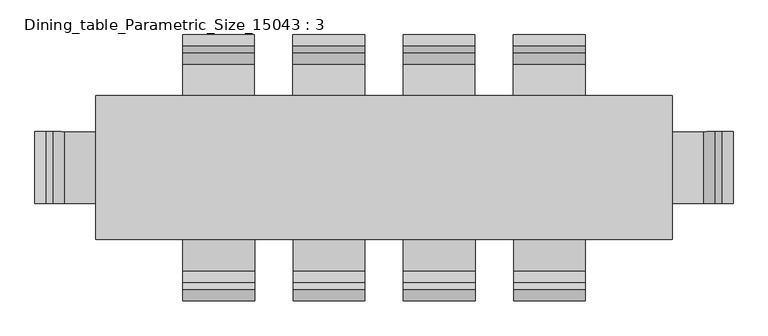
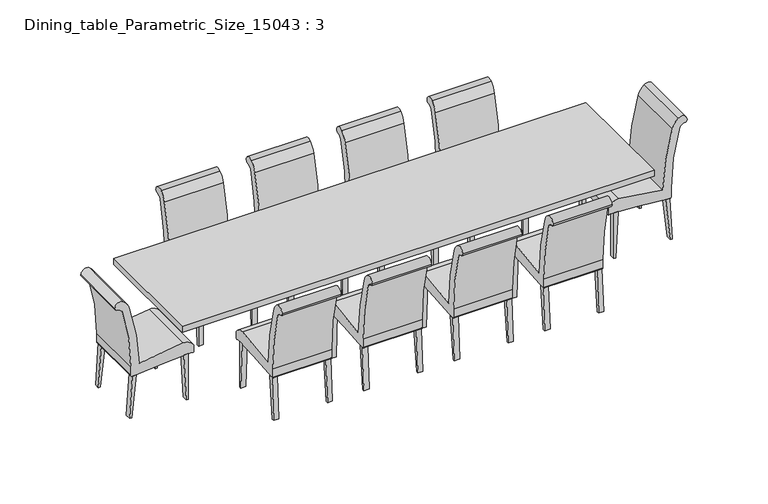
"""IFC4 building model written with IfcOpenShell, lengths in millimetres: furniture geometry, Dining_table_Parametric_Size_15043 : 3."""

from ifc_helpers import new_model, si_unit, point, frame, frame_2d, origin, place, context, project, spatial, polyline, circle_curve, trimmed, segment, composite_curve, outline, extrude, source, transform, mapped, element, save


def dining_table_parametric_size_15043_3_5ca9b808(model_context):
    return source(origin(), model_context, "Body", "SweptSolid", [
        extrude(outline(polyline([(-292.8098174, 0.0), (-312.156828, 373.7391541), (-276.8521088, 373.7391541), (-276.8521088, 0.0), (-292.8098174, 0.0)])), frame((821.4, 0.0, 0.0), z_axis=(1.0, 0.0, 0.0), x_axis=(0.0, 1.0, 0.0)), (0.0, 0.0, 1.0), 38.1),
        extrude(outline(composite_curve([segment(polyline([(-710.0841698, 339.961294), (-678.3341698, 339.961294)]), True, "CONTINUOUS"), segment(trimmed(circle_curve(frame_2d((-4714.5831391, 601.3302132)), 4044.702641), [point((-678.3341698, 339.961294))], [point((-714.8304681, 0.0))], False, "CARTESIAN"), True, "CONTINUOUS"), segment(polyline([(-714.8304681, 0.0), (-730.8247987, 0.0)]), True, "CONTINUOUS"), segment(trimmed(circle_curve(frame_2d((-4796.627411, 418.6630455)), 4087.30102), [point((-730.8247987, 0.0))], [point((-710.0841698, 339.961294))], True, "CARTESIAN"), True, "CONTINUOUS")], self_intersect=False)), frame((822.7642545, 0.0, 0.0), z_axis=(1.0, 0.0, 0.0), x_axis=(0.0, 1.0, 0.0)), (0.0, 0.0, 1.0), 41.6791394),
        extrude(outline(polyline([(-290.2637156, 0.0), (-309.6107262, 373.7391541), (-274.306007, 373.7391541), (-274.306007, 0.0), (-290.2637156, 0.0)])), frame((1240.5, 0.0, 0.0), z_axis=(1.0, 0.0, 0.0), x_axis=(0.0, 1.0, 0.0)), (0.0, 0.0, 1.0), 38.1),
        extrude(outline(composite_curve([segment(polyline([(-710.2334533, 339.961294), (-678.4834533, 339.961294)]), True, "CONTINUOUS"), segment(trimmed(circle_curve(frame_2d((-4714.7324226, 601.3302132)), 4044.702641), [point((-678.4834533, 339.961294))], [point((-714.9797517, 0.0))], False, "CARTESIAN"), True, "CONTINUOUS"), segment(polyline([(-714.9797517, 0.0), (-730.9740822, 0.0)]), True, "CONTINUOUS"), segment(trimmed(circle_curve(frame_2d((-4796.7766946, 418.6630455)), 4087.30102), [point((-730.9740822, 0.0))], [point((-710.2334533, 339.961294))], True, "CARTESIAN"), True, "CONTINUOUS")], self_intersect=False)), frame((1240.5, 0.0, 0.0), z_axis=(1.0, 0.0, 0.0), x_axis=(0.0, 1.0, 0.0)), (0.0, 0.0, 1.0), 38.1),
        extrude(outline(composite_curve([segment(trimmed(circle_curve(frame_2d((-2455.1641625, 418.9322486)), 1733.8120537), [point((-721.3521088, 418.9322486))], [point((-788.5170473, 896.8356186))], True, "CARTESIAN"), True, "CONTINUOUS"), segment(trimmed(circle_curve(frame_2d((-836.5595379, 866.2613731)), 56.9461622), [point((-788.5170473, 896.8356186))], [point((-833.5560291, 923.1282732))], True, "CARTESIAN"), True, "CONTINUOUS"), segment(trimmed(circle_curve(frame_2d((-822.9723933, 942.5682988)), 22.134316), [point((-833.5560291, 923.1282732))], [point((-845.0415591, 944.2653155))], False, "CARTESIAN"), True, "CONTINUOUS"), segment(trimmed(circle_curve(frame_2d((-802.9630897, 941.029676)), 42.2026889), [point((-845.0415591, 944.2653155))], [point((-776.060453, 973.5460579))], False, "CARTESIAN"), True, "CONTINUOUS"), segment(trimmed(circle_curve(frame_2d((-859.9657861, 872.1322861)), 131.6239265), [point((-776.060453, 973.5460579))], [point((-732.0340147, 903.0890285))], False, "CARTESIAN"), True, "CONTINUOUS"), segment(trimmed(circle_curve(frame_2d((-2494.3548845, 379.656989)), 1838.4112565), [point((-732.0340147, 903.0890285))], [point((-656.5387419, 426.4306353))], False, "CARTESIAN"), True, "CONTINUOUS"), segment(trimmed(circle_curve(frame_2d((-123.3478444, -2135.5006423)), 2616.8271636), [point((-656.5387419, 426.4306353))], [point((-316.9758211, 474.1530916))], False, "CARTESIAN"), True, "CONTINUOUS"), segment(trimmed(circle_curve(frame_2d((-310.4852539, 386.6753768)), 87.718174), [point((-316.9758211, 474.1530916))], [point((-232.8604678, 427.5271899))], False, "CARTESIAN"), True, "CONTINUOUS"), segment(polyline([(-232.8604678, 427.5271899), (-232.8604678, 371.8464813), (-237.3505959, 367.3563533), (-247.15219, 373.0153063)]), True, "CONTINUOUS"), segment(trimmed(circle_curve(frame_2d((-291.8347617, -793.4944233)), 1167.3651877), [point((-247.15219, 373.0153063))], [point((-457.2, 362.0988526))], True, "CARTESIAN"), True, "CONTINUOUS"), segment(trimmed(circle_curve(frame_2d((-785.2472905, 2654.5349591)), 2315.7889211), [point((-457.2, 362.0988526))], [point((-710.2334533, 339.961294))], False, "CARTESIAN"), True, "CONTINUOUS"), segment(trimmed(circle_curve(frame_2d((-712.0516896, 349.0822486)), 9.3004191), [point((-710.2334533, 339.961294))], [point((-721.3521088, 349.0822486))], False, "CARTESIAN"), True, "CONTINUOUS"), segment(polyline([(-721.3521088, 349.0822486), (-721.3521088, 418.9322486)]), True, "CONTINUOUS")], self_intersect=False)), frame((822.7642545, 0.0, 0.0), z_axis=(1.0, 0.0, 0.0), x_axis=(0.0, 1.0, 0.0)), (0.0, 0.0, 1.0), 455.8357455),
        extrude(outline(polyline([(-292.8098174, 0.0), (-312.156828, 373.7391541), (-276.8521088, 373.7391541), (-276.8521088, 0.0), (-292.8098174, 0.0)])), frame((121.4, 0.0, 0.0), z_axis=(1.0, 0.0, 0.0), x_axis=(0.0, 1.0, 0.0)), (0.0, 0.0, 1.0), 38.1),
        extrude(outline(composite_curve([segment(polyline([(-710.0841698, 339.961294), (-678.3341698, 339.961294)]), True, "CONTINUOUS"), segment(trimmed(circle_curve(frame_2d((-4714.5831391, 601.3302132)), 4044.702641), [point((-678.3341698, 339.961294))], [point((-714.8304681, 0.0))], False, "CARTESIAN"), True, "CONTINUOUS"), segment(polyline([(-714.8304681, 0.0), (-730.8247987, 0.0)]), True, "CONTINUOUS"), segment(trimmed(circle_curve(frame_2d((-4796.627411, 418.6630455)), 4087.30102), [point((-730.8247987, 0.0))], [point((-710.0841698, 339.961294))], True, "CARTESIAN"), True, "CONTINUOUS")], self_intersect=False)), frame((122.7642545, 0.0, 0.0), z_axis=(1.0, 0.0, 0.0), x_axis=(0.0, 1.0, 0.0)), (0.0, 0.0, 1.0), 41.6791394),
        extrude(outline(polyline([(-290.2637156, 0.0), (-309.6107262, 373.7391541), (-274.306007, 373.7391541), (-274.306007, 0.0), (-290.2637156, 0.0)])), frame((540.5, 0.0, 0.0), z_axis=(1.0, 0.0, 0.0), x_axis=(0.0, 1.0, 0.0)), (0.0, 0.0, 1.0), 38.1),
        extrude(outline(composite_curve([segment(polyline([(-710.2334533, 339.961294), (-678.4834533, 339.961294)]), True, "CONTINUOUS"), segment(trimmed(circle_curve(frame_2d((-4714.7324226, 601.3302132)), 4044.702641), [point((-678.4834533, 339.961294))], [point((-714.9797517, 0.0))], False, "CARTESIAN"), True, "CONTINUOUS"), segment(polyline([(-714.9797517, 0.0), (-730.9740822, 0.0)]), True, "CONTINUOUS"), segment(trimmed(circle_curve(frame_2d((-4796.7766946, 418.6630455)), 4087.30102), [point((-730.9740822, 0.0))], [point((-710.2334533, 339.961294))], True, "CARTESIAN"), True, "CONTINUOUS")], self_intersect=False)), frame((540.5, 0.0, 0.0), z_axis=(1.0, 0.0, 0.0), x_axis=(0.0, 1.0, 0.0)), (0.0, 0.0, 1.0), 38.1),
        extrude(outline(composite_curve([segment(trimmed(circle_curve(frame_2d((-2455.1641625, 418.9322486)), 1733.8120537), [point((-721.3521088, 418.9322486))], [point((-788.5170473, 896.8356186))], True, "CARTESIAN"), True, "CONTINUOUS"), segment(trimmed(circle_curve(frame_2d((-836.5595379, 866.2613731)), 56.9461622), [point((-788.5170473, 896.8356186))], [point((-833.5560291, 923.1282732))], True, "CARTESIAN"), True, "CONTINUOUS"), segment(trimmed(circle_curve(frame_2d((-822.9723933, 942.5682988)), 22.134316), [point((-833.5560291, 923.1282732))], [point((-845.0415591, 944.2653155))], False, "CARTESIAN"), True, "CONTINUOUS"), segment(trimmed(circle_curve(frame_2d((-802.9630897, 941.029676)), 42.2026889), [point((-845.0415591, 944.2653155))], [point((-776.060453, 973.5460579))], False, "CARTESIAN"), True, "CONTINUOUS"), segment(trimmed(circle_curve(frame_2d((-859.9657861, 872.1322861)), 131.6239265), [point((-776.060453, 973.5460579))], [point((-732.0340147, 903.0890285))], False, "CARTESIAN"), True, "CONTINUOUS"), segment(trimmed(circle_curve(frame_2d((-2494.3548845, 379.656989)), 1838.4112565), [point((-732.0340147, 903.0890285))], [point((-656.5387419, 426.4306353))], False, "CARTESIAN"), True, "CONTINUOUS"), segment(trimmed(circle_curve(frame_2d((-123.3478444, -2135.5006423)), 2616.8271636), [point((-656.5387419, 426.4306353))], [point((-316.9758211, 474.1530916))], False, "CARTESIAN"), True, "CONTINUOUS"), segment(trimmed(circle_curve(frame_2d((-310.4852539, 386.6753768)), 87.718174), [point((-316.9758211, 474.1530916))], [point((-232.8604678, 427.5271899))], False, "CARTESIAN"), True, "CONTINUOUS"), segment(polyline([(-232.8604678, 427.5271899), (-232.8604678, 371.8464813), (-237.3505959, 367.3563533), (-247.15219, 373.0153063)]), True, "CONTINUOUS"), segment(trimmed(circle_curve(frame_2d((-291.8347617, -793.4944233)), 1167.3651877), [point((-247.15219, 373.0153063))], [point((-457.2, 362.0988526))], True, "CARTESIAN"), True, "CONTINUOUS"), segment(trimmed(circle_curve(frame_2d((-785.2472905, 2654.5349591)), 2315.7889211), [point((-457.2, 362.0988526))], [point((-710.2334533, 339.961294))], False, "CARTESIAN"), True, "CONTINUOUS"), segment(trimmed(circle_curve(frame_2d((-712.0516896, 349.0822486)), 9.3004191), [point((-710.2334533, 339.961294))], [point((-721.3521088, 349.0822486))], False, "CARTESIAN"), True, "CONTINUOUS"), segment(polyline([(-721.3521088, 349.0822486), (-721.3521088, 418.9322486)]), True, "CONTINUOUS")], self_intersect=False)), frame((122.7642545, 0.0, 0.0), z_axis=(1.0, 0.0, 0.0), x_axis=(0.0, 1.0, 0.0)), (0.0, 0.0, 1.0), 455.8357455),
        extrude(outline(polyline([(292.8098174, 0.0), (276.8521088, 0.0), (276.8521088, 373.7391541), (312.156828, 373.7391541), (292.8098174, 0.0)])), frame((1240.5, 0.0, 0.0), z_axis=(1.0, 0.0, 0.0), x_axis=(0.0, 1.0, 0.0)), (0.0, 0.0, 1.0), 38.1),
        extrude(outline(composite_curve([segment(trimmed(circle_curve(frame_2d((4796.627411, 418.6630455)), 4087.30102), [point((710.0841698, 339.961294))], [point((730.8247987, 0.0))], True, "CARTESIAN"), True, "CONTINUOUS"), segment(polyline([(730.8247987, 0.0), (714.8304681, 0.0)]), True, "CONTINUOUS"), segment(trimmed(circle_curve(frame_2d((4714.5831391, 601.3302132)), 4044.702641), [point((714.8304681, 0.0))], [point((678.3341698, 339.961294))], False, "CARTESIAN"), True, "CONTINUOUS"), segment(polyline([(678.3341698, 339.961294), (710.0841698, 339.961294)]), True, "CONTINUOUS")], self_intersect=False)), frame((1235.5566061, 0.0, 0.0), z_axis=(1.0, 0.0, 0.0), x_axis=(0.0, 1.0, 0.0)), (0.0, 0.0, 1.0), 41.6791394),
        extrude(outline(polyline([(290.2637156, 0.0), (274.306007, 0.0), (274.306007, 373.7391541), (309.6107262, 373.7391541), (290.2637156, 0.0)])), frame((821.4, 0.0, 0.0), z_axis=(1.0, 0.0, 0.0), x_axis=(0.0, 1.0, 0.0)), (0.0, 0.0, 1.0), 38.1),
        extrude(outline(composite_curve([segment(trimmed(circle_curve(frame_2d((4796.7766946, 418.6630455)), 4087.30102), [point((710.2334533, 339.961294))], [point((730.9740822, 0.0))], True, "CARTESIAN"), True, "CONTINUOUS"), segment(polyline([(730.9740822, 0.0), (714.9797517, 0.0)]), True, "CONTINUOUS"), segment(trimmed(circle_curve(frame_2d((4714.7324226, 601.3302132)), 4044.702641), [point((714.9797517, 0.0))], [point((678.4834533, 339.961294))], False, "CARTESIAN"), True, "CONTINUOUS"), segment(polyline([(678.4834533, 339.961294), (710.2334533, 339.961294)]), True, "CONTINUOUS")], self_intersect=False)), frame((821.4, 0.0, 0.0), z_axis=(1.0, 0.0, 0.0), x_axis=(0.0, 1.0, 0.0)), (0.0, 0.0, 1.0), 38.1),
        extrude(outline(composite_curve([segment(polyline([(721.3521088, 418.9322486), (721.3521088, 349.0822486)]), True, "CONTINUOUS"), segment(trimmed(circle_curve(frame_2d((712.0516896, 349.0822486)), 9.3004191), [point((721.3521088, 349.0822486))], [point((710.2334533, 339.961294))], False, "CARTESIAN"), True, "CONTINUOUS"), segment(trimmed(circle_curve(frame_2d((785.2472905, 2654.5349591)), 2315.7889211), [point((710.2334533, 339.961294))], [point((457.2, 362.0988526))], False, "CARTESIAN"), True, "CONTINUOUS"), segment(trimmed(circle_curve(frame_2d((291.8347617, -793.4944233)), 1167.3651877), [point((457.2, 362.0988526))], [point((247.15219, 373.0153063))], True, "CARTESIAN"), True, "CONTINUOUS"), segment(polyline([(247.15219, 373.0153063), (237.3505959, 367.3563533), (232.8604678, 371.8464813), (232.8604678, 427.5271899)]), True, "CONTINUOUS"), segment(trimmed(circle_curve(frame_2d((310.4852539, 386.6753768)), 87.718174), [point((232.8604678, 427.5271899))], [point((316.9758211, 474.1530916))], False, "CARTESIAN"), True, "CONTINUOUS"), segment(trimmed(circle_curve(frame_2d((123.3478444, -2135.5006423)), 2616.8271636), [point((316.9758211, 474.1530916))], [point((656.5387419, 426.4306353))], False, "CARTESIAN"), True, "CONTINUOUS"), segment(trimmed(circle_curve(frame_2d((2494.3548845, 379.656989)), 1838.4112565), [point((656.5387419, 426.4306353))], [point((732.0340147, 903.0890285))], False, "CARTESIAN"), True, "CONTINUOUS"), segment(trimmed(circle_curve(frame_2d((859.9657861, 872.1322861)), 131.6239265), [point((732.0340147, 903.0890285))], [point((776.060453, 973.5460579))], False, "CARTESIAN"), True, "CONTINUOUS"), segment(trimmed(circle_curve(frame_2d((802.9630897, 941.029676)), 42.2026889), [point((776.060453, 973.5460579))], [point((845.0415591, 944.2653155))], False, "CARTESIAN"), True, "CONTINUOUS"), segment(trimmed(circle_curve(frame_2d((822.9723933, 942.5682988)), 22.134316), [point((845.0415591, 944.2653155))], [point((833.5560291, 923.1282732))], False, "CARTESIAN"), True, "CONTINUOUS"), segment(trimmed(circle_curve(frame_2d((836.5595379, 866.2613731)), 56.9461622), [point((833.5560291, 923.1282732))], [point((788.5170473, 896.8356186))], True, "CARTESIAN"), True, "CONTINUOUS"), segment(trimmed(circle_curve(frame_2d((2455.1641625, 418.9322486)), 1733.8120537), [point((788.5170473, 896.8356186))], [point((721.3521088, 418.9322486))], True, "CARTESIAN"), True, "CONTINUOUS")], self_intersect=False)), frame((821.4, 0.0, 0.0), z_axis=(1.0, 0.0, 0.0), x_axis=(0.0, 1.0, 0.0)), (0.0, 0.0, 1.0), 455.8357455),
        extrude(outline(polyline([(292.8098174, 0.0), (276.8521088, 0.0), (276.8521088, 373.7391541), (312.156828, 373.7391541), (292.8098174, 0.0)])), frame((540.5, 0.0, 0.0), z_axis=(1.0, 0.0, 0.0), x_axis=(0.0, 1.0, 0.0)), (0.0, 0.0, 1.0), 38.1),
        extrude(outline(composite_curve([segment(trimmed(circle_curve(frame_2d((4796.627411, 418.6630455)), 4087.30102), [point((710.0841698, 339.961294))], [point((730.8247987, 0.0))], True, "CARTESIAN"), True, "CONTINUOUS"), segment(polyline([(730.8247987, 0.0), (714.8304681, 0.0)]), True, "CONTINUOUS"), segment(trimmed(circle_curve(frame_2d((4714.5831391, 601.3302132)), 4044.702641), [point((714.8304681, 0.0))], [point((678.3341698, 339.961294))], False, "CARTESIAN"), True, "CONTINUOUS"), segment(polyline([(678.3341698, 339.961294), (710.0841698, 339.961294)]), True, "CONTINUOUS")], self_intersect=False)), frame((535.5566061, 0.0, 0.0), z_axis=(1.0, 0.0, 0.0), x_axis=(0.0, 1.0, 0.0)), (0.0, 0.0, 1.0), 41.6791394),
        extrude(outline(polyline([(290.2637156, 0.0), (274.306007, 0.0), (274.306007, 373.7391541), (309.6107262, 373.7391541), (290.2637156, 0.0)])), frame((121.4, 0.0, 0.0), z_axis=(1.0, 0.0, 0.0), x_axis=(0.0, 1.0, 0.0)), (0.0, 0.0, 1.0), 38.1),
        extrude(outline(composite_curve([segment(trimmed(circle_curve(frame_2d((4796.7766946, 418.6630455)), 4087.30102), [point((710.2334533, 339.961294))], [point((730.9740822, 0.0))], True, "CARTESIAN"), True, "CONTINUOUS"), segment(polyline([(730.9740822, 0.0), (714.9797517, 0.0)]), True, "CONTINUOUS"), segment(trimmed(circle_curve(frame_2d((4714.7324226, 601.3302132)), 4044.702641), [point((714.9797517, 0.0))], [point((678.4834533, 339.961294))], False, "CARTESIAN"), True, "CONTINUOUS"), segment(polyline([(678.4834533, 339.961294), (710.2334533, 339.961294)]), True, "CONTINUOUS")], self_intersect=False)), frame((121.4, 0.0, 0.0), z_axis=(1.0, 0.0, 0.0), x_axis=(0.0, 1.0, 0.0)), (0.0, 0.0, 1.0), 38.1),
        extrude(outline(composite_curve([segment(polyline([(721.3521088, 418.9322486), (721.3521088, 349.0822486)]), True, "CONTINUOUS"), segment(trimmed(circle_curve(frame_2d((712.0516896, 349.0822486)), 9.3004191), [point((721.3521088, 349.0822486))], [point((710.2334533, 339.961294))], False, "CARTESIAN"), True, "CONTINUOUS"), segment(trimmed(circle_curve(frame_2d((785.2472905, 2654.5349591)), 2315.7889211), [point((710.2334533, 339.961294))], [point((457.2, 362.0988526))], False, "CARTESIAN"), True, "CONTINUOUS"), segment(trimmed(circle_curve(frame_2d((291.8347617, -793.4944233)), 1167.3651877), [point((457.2, 362.0988526))], [point((247.15219, 373.0153063))], True, "CARTESIAN"), True, "CONTINUOUS"), segment(polyline([(247.15219, 373.0153063), (237.3505959, 367.3563533), (232.8604678, 371.8464813), (232.8604678, 427.5271899)]), True, "CONTINUOUS"), segment(trimmed(circle_curve(frame_2d((310.4852539, 386.6753768)), 87.718174), [point((232.8604678, 427.5271899))], [point((316.9758211, 474.1530916))], False, "CARTESIAN"), True, "CONTINUOUS"), segment(trimmed(circle_curve(frame_2d((123.3478444, -2135.5006423)), 2616.8271636), [point((316.9758211, 474.1530916))], [point((656.5387419, 426.4306353))], False, "CARTESIAN"), True, "CONTINUOUS"), segment(trimmed(circle_curve(frame_2d((2494.3548845, 379.656989)), 1838.4112565), [point((656.5387419, 426.4306353))], [point((732.0340147, 903.0890285))], False, "CARTESIAN"), True, "CONTINUOUS"), segment(trimmed(circle_curve(frame_2d((859.9657861, 872.1322861)), 131.6239265), [point((732.0340147, 903.0890285))], [point((776.060453, 973.5460579))], False, "CARTESIAN"), True, "CONTINUOUS"), segment(trimmed(circle_curve(frame_2d((802.9630897, 941.029676)), 42.2026889), [point((776.060453, 973.5460579))], [point((845.0415591, 944.2653155))], False, "CARTESIAN"), True, "CONTINUOUS"), segment(trimmed(circle_curve(frame_2d((822.9723933, 942.5682988)), 22.134316), [point((845.0415591, 944.2653155))], [point((833.5560291, 923.1282732))], False, "CARTESIAN"), True, "CONTINUOUS"), segment(trimmed(circle_curve(frame_2d((836.5595379, 866.2613731)), 56.9461622), [point((833.5560291, 923.1282732))], [point((788.5170473, 896.8356186))], True, "CARTESIAN"), True, "CONTINUOUS"), segment(trimmed(circle_curve(frame_2d((2455.1641625, 418.9322486)), 1733.8120537), [point((788.5170473, 896.8356186))], [point((721.3521088, 418.9322486))], True, "CARTESIAN"), True, "CONTINUOUS")], self_intersect=False)), frame((121.4, 0.0, 0.0), z_axis=(1.0, 0.0, 0.0), x_axis=(0.0, 1.0, 0.0)), (0.0, 0.0, 1.0), 455.8357455),
        extrude(outline(polyline([(-292.8098174, 0.0), (-312.156828, 373.7391541), (-276.8521088, 373.7391541), (-276.8521088, 0.0), (-292.8098174, 0.0)])), frame((-578.6, 0.0, 0.0), z_axis=(1.0, 0.0, 0.0), x_axis=(0.0, 1.0, 0.0)), (0.0, 0.0, 1.0), 38.1),
        extrude(outline(composite_curve([segment(polyline([(-710.0841698, 339.961294), (-678.3341698, 339.961294)]), True, "CONTINUOUS"), segment(trimmed(circle_curve(frame_2d((-4714.5831391, 601.3302132)), 4044.702641), [point((-678.3341698, 339.961294))], [point((-714.8304681, 0.0))], False, "CARTESIAN"), True, "CONTINUOUS"), segment(polyline([(-714.8304681, 0.0), (-730.8247987, 0.0)]), True, "CONTINUOUS"), segment(trimmed(circle_curve(frame_2d((-4796.627411, 418.6630455)), 4087.30102), [point((-730.8247987, 0.0))], [point((-710.0841698, 339.961294))], True, "CARTESIAN"), True, "CONTINUOUS")], self_intersect=False)), frame((-577.2357455, 0.0, 0.0), z_axis=(1.0, 0.0, 0.0), x_axis=(0.0, 1.0, 0.0)), (0.0, 0.0, 1.0), 41.6791394),
        extrude(outline(polyline([(-290.2637156, 0.0), (-309.6107262, 373.7391541), (-274.306007, 373.7391541), (-274.306007, 0.0), (-290.2637156, 0.0)])), frame((-159.5, 0.0, 0.0), z_axis=(1.0, 0.0, 0.0), x_axis=(0.0, 1.0, 0.0)), (0.0, 0.0, 1.0), 38.1),
        extrude(outline(composite_curve([segment(polyline([(-710.2334533, 339.961294), (-678.4834533, 339.961294)]), True, "CONTINUOUS"), segment(trimmed(circle_curve(frame_2d((-4714.7324226, 601.3302132)), 4044.702641), [point((-678.4834533, 339.961294))], [point((-714.9797517, 0.0))], False, "CARTESIAN"), True, "CONTINUOUS"), segment(polyline([(-714.9797517, 0.0), (-730.9740822, 0.0)]), True, "CONTINUOUS"), segment(trimmed(circle_curve(frame_2d((-4796.7766946, 418.6630455)), 4087.30102), [point((-730.9740822, 0.0))], [point((-710.2334533, 339.961294))], True, "CARTESIAN"), True, "CONTINUOUS")], self_intersect=False)), frame((-159.5, 0.0, 0.0), z_axis=(1.0, 0.0, 0.0), x_axis=(0.0, 1.0, 0.0)), (0.0, 0.0, 1.0), 38.1),
        extrude(outline(composite_curve([segment(trimmed(circle_curve(frame_2d((-2455.1641625, 418.9322486)), 1733.8120537), [point((-721.3521088, 418.9322486))], [point((-788.5170473, 896.8356186))], True, "CARTESIAN"), True, "CONTINUOUS"), segment(trimmed(circle_curve(frame_2d((-836.5595379, 866.2613731)), 56.9461622), [point((-788.5170473, 896.8356186))], [point((-833.5560291, 923.1282732))], True, "CARTESIAN"), True, "CONTINUOUS"), segment(trimmed(circle_curve(frame_2d((-822.9723933, 942.5682988)), 22.134316), [point((-833.5560291, 923.1282732))], [point((-845.0415591, 944.2653155))], False, "CARTESIAN"), True, "CONTINUOUS"), segment(trimmed(circle_curve(frame_2d((-802.9630897, 941.029676)), 42.2026889), [point((-845.0415591, 944.2653155))], [point((-776.060453, 973.5460579))], False, "CARTESIAN"), True, "CONTINUOUS"), segment(trimmed(circle_curve(frame_2d((-859.9657861, 872.1322861)), 131.6239265), [point((-776.060453, 973.5460579))], [point((-732.0340147, 903.0890285))], False, "CARTESIAN"), True, "CONTINUOUS"), segment(trimmed(circle_curve(frame_2d((-2494.3548845, 379.656989)), 1838.4112565), [point((-732.0340147, 903.0890285))], [point((-656.5387419, 426.4306353))], False, "CARTESIAN"), True, "CONTINUOUS"), segment(trimmed(circle_curve(frame_2d((-123.3478444, -2135.5006423)), 2616.8271636), [point((-656.5387419, 426.4306353))], [point((-316.9758211, 474.1530916))], False, "CARTESIAN"), True, "CONTINUOUS"), segment(trimmed(circle_curve(frame_2d((-310.4852539, 386.6753768)), 87.718174), [point((-316.9758211, 474.1530916))], [point((-232.8604678, 427.5271899))], False, "CARTESIAN"), True, "CONTINUOUS"), segment(polyline([(-232.8604678, 427.5271899), (-232.8604678, 371.8464813), (-237.3505959, 367.3563533), (-247.15219, 373.0153063)]), True, "CONTINUOUS"), segment(trimmed(circle_curve(frame_2d((-291.8347617, -793.4944233)), 1167.3651877), [point((-247.15219, 373.0153063))], [point((-457.2, 362.0988526))], True, "CARTESIAN"), True, "CONTINUOUS"), segment(trimmed(circle_curve(frame_2d((-785.2472905, 2654.5349591)), 2315.7889211), [point((-457.2, 362.0988526))], [point((-710.2334533, 339.961294))], False, "CARTESIAN"), True, "CONTINUOUS"), segment(trimmed(circle_curve(frame_2d((-712.0516896, 349.0822486)), 9.3004191), [point((-710.2334533, 339.961294))], [point((-721.3521088, 349.0822486))], False, "CARTESIAN"), True, "CONTINUOUS"), segment(polyline([(-721.3521088, 349.0822486), (-721.3521088, 418.9322486)]), True, "CONTINUOUS")], self_intersect=False)), frame((-577.2357455, 0.0, 0.0), z_axis=(1.0, 0.0, 0.0), x_axis=(0.0, 1.0, 0.0)), (0.0, 0.0, 1.0), 455.8357455),
        extrude(outline(polyline([(-292.8098174, 0.0), (-312.156828, 373.7391541), (-276.8521088, 373.7391541), (-276.8521088, 0.0), (-292.8098174, 0.0)])), frame((-1278.6, 0.0, 0.0), z_axis=(1.0, 0.0, 0.0), x_axis=(0.0, 1.0, 0.0)), (0.0, 0.0, 1.0), 38.1),
        extrude(outline(composite_curve([segment(polyline([(-710.0841698, 339.961294), (-678.3341698, 339.961294)]), True, "CONTINUOUS"), segment(trimmed(circle_curve(frame_2d((-4714.5831391, 601.3302132)), 4044.702641), [point((-678.3341698, 339.961294))], [point((-714.8304681, 0.0))], False, "CARTESIAN"), True, "CONTINUOUS"), segment(polyline([(-714.8304681, 0.0), (-730.8247987, 0.0)]), True, "CONTINUOUS"), segment(trimmed(circle_curve(frame_2d((-4796.627411, 418.6630455)), 4087.30102), [point((-730.8247987, 0.0))], [point((-710.0841698, 339.961294))], True, "CARTESIAN"), True, "CONTINUOUS")], self_intersect=False)), frame((-1277.2357455, 0.0, 0.0), z_axis=(1.0, 0.0, 0.0), x_axis=(0.0, 1.0, 0.0)), (0.0, 0.0, 1.0), 41.6791394),
        extrude(outline(polyline([(-290.2637156, 0.0), (-309.6107262, 373.7391541), (-274.306007, 373.7391541), (-274.306007, 0.0), (-290.2637156, 0.0)])), frame((-859.5, 0.0, 0.0), z_axis=(1.0, 0.0, 0.0), x_axis=(0.0, 1.0, 0.0)), (0.0, 0.0, 1.0), 38.1),
        extrude(outline(composite_curve([segment(polyline([(-710.2334533, 339.961294), (-678.4834533, 339.961294)]), True, "CONTINUOUS"), segment(trimmed(circle_curve(frame_2d((-4714.7324226, 601.3302132)), 4044.702641), [point((-678.4834533, 339.961294))], [point((-714.9797517, 0.0))], False, "CARTESIAN"), True, "CONTINUOUS"), segment(polyline([(-714.9797517, 0.0), (-730.9740822, 0.0)]), True, "CONTINUOUS"), segment(trimmed(circle_curve(frame_2d((-4796.7766946, 418.6630455)), 4087.30102), [point((-730.9740822, 0.0))], [point((-710.2334533, 339.961294))], True, "CARTESIAN"), True, "CONTINUOUS")], self_intersect=False)), frame((-859.5, 0.0, 0.0), z_axis=(1.0, 0.0, 0.0), x_axis=(0.0, 1.0, 0.0)), (0.0, 0.0, 1.0), 38.1),
        extrude(outline(composite_curve([segment(trimmed(circle_curve(frame_2d((-2455.1641625, 418.9322486)), 1733.8120537), [point((-721.3521088, 418.9322486))], [point((-788.5170473, 896.8356186))], True, "CARTESIAN"), True, "CONTINUOUS"), segment(trimmed(circle_curve(frame_2d((-836.5595379, 866.2613731)), 56.9461622), [point((-788.5170473, 896.8356186))], [point((-833.5560291, 923.1282732))], True, "CARTESIAN"), True, "CONTINUOUS"), segment(trimmed(circle_curve(frame_2d((-822.9723933, 942.5682988)), 22.134316), [point((-833.5560291, 923.1282732))], [point((-845.0415591, 944.2653155))], False, "CARTESIAN"), True, "CONTINUOUS"), segment(trimmed(circle_curve(frame_2d((-802.9630897, 941.029676)), 42.2026889), [point((-845.0415591, 944.2653155))], [point((-776.060453, 973.5460579))], False, "CARTESIAN"), True, "CONTINUOUS"), segment(trimmed(circle_curve(frame_2d((-859.9657861, 872.1322861)), 131.6239265), [point((-776.060453, 973.5460579))], [point((-732.0340147, 903.0890285))], False, "CARTESIAN"), True, "CONTINUOUS"), segment(trimmed(circle_curve(frame_2d((-2494.3548845, 379.656989)), 1838.4112565), [point((-732.0340147, 903.0890285))], [point((-656.5387419, 426.4306353))], False, "CARTESIAN"), True, "CONTINUOUS"), segment(trimmed(circle_curve(frame_2d((-123.3478444, -2135.5006423)), 2616.8271636), [point((-656.5387419, 426.4306353))], [point((-316.9758211, 474.1530916))], False, "CARTESIAN"), True, "CONTINUOUS"), segment(trimmed(circle_curve(frame_2d((-310.4852539, 386.6753768)), 87.718174), [point((-316.9758211, 474.1530916))], [point((-232.8604678, 427.5271899))], False, "CARTESIAN"), True, "CONTINUOUS"), segment(polyline([(-232.8604678, 427.5271899), (-232.8604678, 371.8464813), (-237.3505959, 367.3563533), (-247.15219, 373.0153063)]), True, "CONTINUOUS"), segment(trimmed(circle_curve(frame_2d((-291.8347617, -793.4944233)), 1167.3651877), [point((-247.15219, 373.0153063))], [point((-457.2, 362.0988526))], True, "CARTESIAN"), True, "CONTINUOUS"), segment(trimmed(circle_curve(frame_2d((-785.2472905, 2654.5349591)), 2315.7889211), [point((-457.2, 362.0988526))], [point((-710.2334533, 339.961294))], False, "CARTESIAN"), True, "CONTINUOUS"), segment(trimmed(circle_curve(frame_2d((-712.0516896, 349.0822486)), 9.3004191), [point((-710.2334533, 339.961294))], [point((-721.3521088, 349.0822486))], False, "CARTESIAN"), True, "CONTINUOUS"), segment(polyline([(-721.3521088, 349.0822486), (-721.3521088, 418.9322486)]), True, "CONTINUOUS")], self_intersect=False)), frame((-1277.2357455, 0.0, 0.0), z_axis=(1.0, 0.0, 0.0), x_axis=(0.0, 1.0, 0.0)), (0.0, 0.0, 1.0), 455.8357455),
        extrude(outline(polyline([(292.8098174, 0.0), (276.8521088, 0.0), (276.8521088, 373.7391541), (312.156828, 373.7391541), (292.8098174, 0.0)])), frame((-159.5, 0.0, 0.0), z_axis=(1.0, 0.0, 0.0), x_axis=(0.0, 1.0, 0.0)), (0.0, 0.0, 1.0), 38.1),
        extrude(outline(composite_curve([segment(trimmed(circle_curve(frame_2d((4796.627411, 418.6630455)), 4087.30102), [point((710.0841698, 339.961294))], [point((730.8247987, 0.0))], True, "CARTESIAN"), True, "CONTINUOUS"), segment(polyline([(730.8247987, 0.0), (714.8304681, 0.0)]), True, "CONTINUOUS"), segment(trimmed(circle_curve(frame_2d((4714.5831391, 601.3302132)), 4044.702641), [point((714.8304681, 0.0))], [point((678.3341698, 339.961294))], False, "CARTESIAN"), True, "CONTINUOUS"), segment(polyline([(678.3341698, 339.961294), (710.0841698, 339.961294)]), True, "CONTINUOUS")], self_intersect=False)), frame((-164.4433939, 0.0, 0.0), z_axis=(1.0, 0.0, 0.0), x_axis=(0.0, 1.0, 0.0)), (0.0, 0.0, 1.0), 41.6791394),
        extrude(outline(polyline([(290.2637156, 0.0), (274.306007, 0.0), (274.306007, 373.7391541), (309.6107262, 373.7391541), (290.2637156, 0.0)])), frame((-578.6, 0.0, 0.0), z_axis=(1.0, 0.0, 0.0), x_axis=(0.0, 1.0, 0.0)), (0.0, 0.0, 1.0), 38.1),
        extrude(outline(composite_curve([segment(trimmed(circle_curve(frame_2d((4796.7766946, 418.6630455)), 4087.30102), [point((710.2334533, 339.961294))], [point((730.9740822, 0.0))], True, "CARTESIAN"), True, "CONTINUOUS"), segment(polyline([(730.9740822, 0.0), (714.9797517, 0.0)]), True, "CONTINUOUS"), segment(trimmed(circle_curve(frame_2d((4714.7324226, 601.3302132)), 4044.702641), [point((714.9797517, 0.0))], [point((678.4834533, 339.961294))], False, "CARTESIAN"), True, "CONTINUOUS"), segment(polyline([(678.4834533, 339.961294), (710.2334533, 339.961294)]), True, "CONTINUOUS")], self_intersect=False)), frame((-578.6, 0.0, 0.0), z_axis=(1.0, 0.0, 0.0), x_axis=(0.0, 1.0, 0.0)), (0.0, 0.0, 1.0), 38.1),
        extrude(outline(composite_curve([segment(polyline([(721.3521088, 418.9322486), (721.3521088, 349.0822486)]), True, "CONTINUOUS"), segment(trimmed(circle_curve(frame_2d((712.0516896, 349.0822486)), 9.3004191), [point((721.3521088, 349.0822486))], [point((710.2334533, 339.961294))], False, "CARTESIAN"), True, "CONTINUOUS"), segment(trimmed(circle_curve(frame_2d((785.2472905, 2654.5349591)), 2315.7889211), [point((710.2334533, 339.961294))], [point((457.2, 362.0988526))], False, "CARTESIAN"), True, "CONTINUOUS"), segment(trimmed(circle_curve(frame_2d((291.8347617, -793.4944233)), 1167.3651877), [point((457.2, 362.0988526))], [point((247.15219, 373.0153063))], True, "CARTESIAN"), True, "CONTINUOUS"), segment(polyline([(247.15219, 373.0153063), (237.3505959, 367.3563533), (232.8604678, 371.8464813), (232.8604678, 427.5271899)]), True, "CONTINUOUS"), segment(trimmed(circle_curve(frame_2d((310.4852539, 386.6753768)), 87.718174), [point((232.8604678, 427.5271899))], [point((316.9758211, 474.1530916))], False, "CARTESIAN"), True, "CONTINUOUS"), segment(trimmed(circle_curve(frame_2d((123.3478444, -2135.5006423)), 2616.8271636), [point((316.9758211, 474.1530916))], [point((656.5387419, 426.4306353))], False, "CARTESIAN"), True, "CONTINUOUS"), segment(trimmed(circle_curve(frame_2d((2494.3548845, 379.656989)), 1838.4112565), [point((656.5387419, 426.4306353))], [point((732.0340147, 903.0890285))], False, "CARTESIAN"), True, "CONTINUOUS"), segment(trimmed(circle_curve(frame_2d((859.9657861, 872.1322861)), 131.6239265), [point((732.0340147, 903.0890285))], [point((776.060453, 973.5460579))], False, "CARTESIAN"), True, "CONTINUOUS"), segment(trimmed(circle_curve(frame_2d((802.9630897, 941.029676)), 42.2026889), [point((776.060453, 973.5460579))], [point((845.0415591, 944.2653155))], False, "CARTESIAN"), True, "CONTINUOUS"), segment(trimmed(circle_curve(frame_2d((822.9723933, 942.5682988)), 22.134316), [point((845.0415591, 944.2653155))], [point((833.5560291, 923.1282732))], False, "CARTESIAN"), True, "CONTINUOUS"), segment(trimmed(circle_curve(frame_2d((836.5595379, 866.2613731)), 56.9461622), [point((833.5560291, 923.1282732))], [point((788.5170473, 896.8356186))], True, "CARTESIAN"), True, "CONTINUOUS"), segment(trimmed(circle_curve(frame_2d((2455.1641625, 418.9322486)), 1733.8120537), [point((788.5170473, 896.8356186))], [point((721.3521088, 418.9322486))], True, "CARTESIAN"), True, "CONTINUOUS")], self_intersect=False)), frame((-578.6, 0.0, 0.0), z_axis=(1.0, 0.0, 0.0), x_axis=(0.0, 1.0, 0.0)), (0.0, 0.0, 1.0), 455.8357455),
        extrude(outline(polyline([(292.8098174, 0.0), (276.8521088, 0.0), (276.8521088, 373.7391541), (312.156828, 373.7391541), (292.8098174, 0.0)])), frame((-859.5, 0.0, 0.0), z_axis=(1.0, 0.0, 0.0), x_axis=(0.0, 1.0, 0.0)), (0.0, 0.0, 1.0), 38.1),
        extrude(outline(composite_curve([segment(trimmed(circle_curve(frame_2d((4796.627411, 418.6630455)), 4087.30102), [point((710.0841698, 339.961294))], [point((730.8247987, 0.0))], True, "CARTESIAN"), True, "CONTINUOUS"), segment(polyline([(730.8247987, 0.0), (714.8304681, 0.0)]), True, "CONTINUOUS"), segment(trimmed(circle_curve(frame_2d((4714.5831391, 601.3302132)), 4044.702641), [point((714.8304681, 0.0))], [point((678.3341698, 339.961294))], False, "CARTESIAN"), True, "CONTINUOUS"), segment(polyline([(678.3341698, 339.961294), (710.0841698, 339.961294)]), True, "CONTINUOUS")], self_intersect=False)), frame((-864.4433939, 0.0, 0.0), z_axis=(1.0, 0.0, 0.0), x_axis=(0.0, 1.0, 0.0)), (0.0, 0.0, 1.0), 41.6791394),
        extrude(outline(polyline([(290.2637156, 0.0), (274.306007, 0.0), (274.306007, 373.7391541), (309.6107262, 373.7391541), (290.2637156, 0.0)])), frame((-1278.6, 0.0, 0.0), z_axis=(1.0, 0.0, 0.0), x_axis=(0.0, 1.0, 0.0)), (0.0, 0.0, 1.0), 38.1),
        extrude(outline(composite_curve([segment(trimmed(circle_curve(frame_2d((4796.7766946, 418.6630455)), 4087.30102), [point((710.2334533, 339.961294))], [point((730.9740822, 0.0))], True, "CARTESIAN"), True, "CONTINUOUS"), segment(polyline([(730.9740822, 0.0), (714.9797517, 0.0)]), True, "CONTINUOUS"), segment(trimmed(circle_curve(frame_2d((4714.7324226, 601.3302132)), 4044.702641), [point((714.9797517, 0.0))], [point((678.4834533, 339.961294))], False, "CARTESIAN"), True, "CONTINUOUS"), segment(polyline([(678.4834533, 339.961294), (710.2334533, 339.961294)]), True, "CONTINUOUS")], self_intersect=False)), frame((-1278.6, 0.0, 0.0), z_axis=(1.0, 0.0, 0.0), x_axis=(0.0, 1.0, 0.0)), (0.0, 0.0, 1.0), 38.1),
        extrude(outline(composite_curve([segment(polyline([(721.3521088, 418.9322486), (721.3521088, 349.0822486)]), True, "CONTINUOUS"), segment(trimmed(circle_curve(frame_2d((712.0516896, 349.0822486)), 9.3004191), [point((721.3521088, 349.0822486))], [point((710.2334533, 339.961294))], False, "CARTESIAN"), True, "CONTINUOUS"), segment(trimmed(circle_curve(frame_2d((785.2472905, 2654.5349591)), 2315.7889211), [point((710.2334533, 339.961294))], [point((457.2, 362.0988526))], False, "CARTESIAN"), True, "CONTINUOUS"), segment(trimmed(circle_curve(frame_2d((291.8347617, -793.4944233)), 1167.3651877), [point((457.2, 362.0988526))], [point((247.15219, 373.0153063))], True, "CARTESIAN"), True, "CONTINUOUS"), segment(polyline([(247.15219, 373.0153063), (237.3505959, 367.3563533), (232.8604678, 371.8464813), (232.8604678, 427.5271899)]), True, "CONTINUOUS"), segment(trimmed(circle_curve(frame_2d((310.4852539, 386.6753768)), 87.718174), [point((232.8604678, 427.5271899))], [point((316.9758211, 474.1530916))], False, "CARTESIAN"), True, "CONTINUOUS"), segment(trimmed(circle_curve(frame_2d((123.3478444, -2135.5006423)), 2616.8271636), [point((316.9758211, 474.1530916))], [point((656.5387419, 426.4306353))], False, "CARTESIAN"), True, "CONTINUOUS"), segment(trimmed(circle_curve(frame_2d((2494.3548845, 379.656989)), 1838.4112565), [point((656.5387419, 426.4306353))], [point((732.0340147, 903.0890285))], False, "CARTESIAN"), True, "CONTINUOUS"), segment(trimmed(circle_curve(frame_2d((859.9657861, 872.1322861)), 131.6239265), [point((732.0340147, 903.0890285))], [point((776.060453, 973.5460579))], False, "CARTESIAN"), True, "CONTINUOUS"), segment(trimmed(circle_curve(frame_2d((802.9630897, 941.029676)), 42.2026889), [point((776.060453, 973.5460579))], [point((845.0415591, 944.2653155))], False, "CARTESIAN"), True, "CONTINUOUS"), segment(trimmed(circle_curve(frame_2d((822.9723933, 942.5682988)), 22.134316), [point((845.0415591, 944.2653155))], [point((833.5560291, 923.1282732))], False, "CARTESIAN"), True, "CONTINUOUS"), segment(trimmed(circle_curve(frame_2d((836.5595379, 866.2613731)), 56.9461622), [point((833.5560291, 923.1282732))], [point((788.5170473, 896.8356186))], True, "CARTESIAN"), True, "CONTINUOUS"), segment(trimmed(circle_curve(frame_2d((2455.1641625, 418.9322486)), 1733.8120537), [point((788.5170473, 896.8356186))], [point((721.3521088, 418.9322486))], True, "CARTESIAN"), True, "CONTINUOUS")], self_intersect=False)), frame((-1278.6, 0.0, 0.0), z_axis=(1.0, 0.0, 0.0), x_axis=(0.0, 1.0, 0.0)), (0.0, 0.0, 1.0), 455.8357455),
        extrude(outline(polyline([(0.0, -1664.4098174), (0.0, -1648.4521088), (373.7391541, -1648.4521088), (373.7391541, -1683.756828), (0.0, -1664.4098174)])), frame((0.0, -228.6, 0.0), z_axis=(0.0, 1.0, 0.0), x_axis=(0.0, 0.0, 1.0)), (0.0, 0.0, 1.0), 38.1),
        extrude(outline(composite_curve([segment(trimmed(circle_curve(frame_2d((418.6630455, -6168.227411)), 4087.30102), [point((339.961294, -2081.6841698))], [point((0.0, -2102.4247987))], True, "CARTESIAN"), True, "CONTINUOUS"), segment(polyline([(0.0, -2102.4247987), (0.0, -2086.4304681)]), True, "CONTINUOUS"), segment(trimmed(circle_curve(frame_2d((601.3302132, -6086.1831391)), 4044.702641), [point((0.0, -2086.4304681))], [point((339.961294, -2049.9341698))], False, "CARTESIAN"), True, "CONTINUOUS"), segment(polyline([(339.961294, -2049.9341698), (339.961294, -2081.6841698)]), True, "CONTINUOUS")], self_intersect=False)), frame((0.0, -227.2357455, 0.0), z_axis=(0.0, 1.0, 0.0), x_axis=(0.0, 0.0, 1.0)), (0.0, 0.0, 1.0), 41.6791394),
        extrude(outline(polyline([(0.0, -1661.8637156), (0.0, -1645.906007), (373.7391541, -1645.906007), (373.7391541, -1681.2107262), (0.0, -1661.8637156)])), frame((0.0, 190.5, 0.0), z_axis=(0.0, 1.0, 0.0), x_axis=(0.0, 0.0, 1.0)), (0.0, 0.0, 1.0), 38.1),
        extrude(outline(composite_curve([segment(trimmed(circle_curve(frame_2d((418.6630455, -6168.3766946)), 4087.30102), [point((339.961294, -2081.8334533))], [point((0.0, -2102.5740822))], True, "CARTESIAN"), True, "CONTINUOUS"), segment(polyline([(0.0, -2102.5740822), (0.0, -2086.5797517)]), True, "CONTINUOUS"), segment(trimmed(circle_curve(frame_2d((601.3302132, -6086.3324226)), 4044.702641), [point((0.0, -2086.5797517))], [point((339.961294, -2050.0834533))], False, "CARTESIAN"), True, "CONTINUOUS"), segment(polyline([(339.961294, -2050.0834533), (339.961294, -2081.8334533)]), True, "CONTINUOUS")], self_intersect=False)), frame((0.0, 190.5, 0.0), z_axis=(0.0, 1.0, 0.0), x_axis=(0.0, 0.0, 1.0)), (0.0, 0.0, 1.0), 38.1),
        extrude(outline(composite_curve([segment(polyline([(418.9322486, -2092.9521088), (349.0822486, -2092.9521088)]), True, "CONTINUOUS"), segment(trimmed(circle_curve(frame_2d((349.0822486, -2083.6516896)), 9.3004191), [point((349.0822486, -2092.9521088))], [point((339.961294, -2081.8334533))], False, "CARTESIAN"), True, "CONTINUOUS"), segment(trimmed(circle_curve(frame_2d((2654.5349591, -2156.8472905)), 2315.7889211), [point((339.961294, -2081.8334533))], [point((362.0988526, -1828.8))], False, "CARTESIAN"), True, "CONTINUOUS"), segment(trimmed(circle_curve(frame_2d((-793.4944233, -1663.4347617)), 1167.3651877), [point((362.0988526, -1828.8))], [point((373.0153063, -1618.75219))], True, "CARTESIAN"), True, "CONTINUOUS"), segment(polyline([(373.0153063, -1618.75219), (367.3563533, -1608.9505959), (371.8464813, -1604.4604678), (427.5271899, -1604.4604678)]), True, "CONTINUOUS"), segment(trimmed(circle_curve(frame_2d((386.6753768, -1682.0852539)), 87.718174), [point((427.5271899, -1604.4604678))], [point((474.1530916, -1688.5758211))], False, "CARTESIAN"), True, "CONTINUOUS"), segment(trimmed(circle_curve(frame_2d((-2135.5006423, -1494.9478444)), 2616.8271636), [point((474.1530916, -1688.5758211))], [point((426.4306353, -2028.1387419))], False, "CARTESIAN"), True, "CONTINUOUS"), segment(trimmed(circle_curve(frame_2d((379.656989, -3865.9548845)), 1838.4112565), [point((426.4306353, -2028.1387419))], [point((903.0890285, -2103.6340147))], False, "CARTESIAN"), True, "CONTINUOUS"), segment(trimmed(circle_curve(frame_2d((872.1322861, -2231.5657861)), 131.6239265), [point((903.0890285, -2103.6340147))], [point((973.5460579, -2147.660453))], False, "CARTESIAN"), True, "CONTINUOUS"), segment(trimmed(circle_curve(frame_2d((941.029676, -2174.5630897)), 42.2026889), [point((973.5460579, -2147.660453))], [point((944.2653155, -2216.6415591))], False, "CARTESIAN"), True, "CONTINUOUS"), segment(trimmed(circle_curve(frame_2d((942.5682988, -2194.5723933)), 22.134316), [point((944.2653155, -2216.6415591))], [point((923.1282732, -2205.1560291))], False, "CARTESIAN"), True, "CONTINUOUS"), segment(trimmed(circle_curve(frame_2d((866.2613731, -2208.1595379)), 56.9461622), [point((923.1282732, -2205.1560291))], [point((896.8356186, -2160.1170473))], True, "CARTESIAN"), True, "CONTINUOUS"), segment(trimmed(circle_curve(frame_2d((418.9322486, -3826.7641625)), 1733.8120537), [point((896.8356186, -2160.1170473))], [point((418.9322486, -2092.9521088))], True, "CARTESIAN"), True, "CONTINUOUS")], self_intersect=False)), frame((0.0, -227.2357455, 0.0), z_axis=(0.0, 1.0, 0.0), x_axis=(0.0, 0.0, 1.0)), (0.0, 0.0, 1.0), 455.8357455),
        extrude(outline(polyline([(0.0, 1664.4098174), (373.7391541, 1683.756828), (373.7391541, 1648.4521088), (0.0, 1648.4521088), (0.0, 1664.4098174)])), frame((0.0, -228.6, 0.0), z_axis=(0.0, 1.0, 0.0), x_axis=(0.0, 0.0, 1.0)), (0.0, 0.0, 1.0), 38.1),
        extrude(outline(composite_curve([segment(polyline([(339.961294, 2081.6841698), (339.961294, 2049.9341698)]), True, "CONTINUOUS"), segment(trimmed(circle_curve(frame_2d((601.3302132, 6086.1831391)), 4044.702641), [point((339.961294, 2049.9341698))], [point((0.0, 2086.4304681))], False, "CARTESIAN"), True, "CONTINUOUS"), segment(polyline([(0.0, 2086.4304681), (0.0, 2102.4247987)]), True, "CONTINUOUS"), segment(trimmed(circle_curve(frame_2d((418.6630455, 6168.227411)), 4087.30102), [point((0.0, 2102.4247987))], [point((339.961294, 2081.6841698))], True, "CARTESIAN"), True, "CONTINUOUS")], self_intersect=False)), frame((0.0, -227.2357455, 0.0), z_axis=(0.0, 1.0, 0.0), x_axis=(0.0, 0.0, 1.0)), (0.0, 0.0, 1.0), 41.6791394),
        extrude(outline(polyline([(0.0, 1661.8637156), (373.7391541, 1681.2107262), (373.7391541, 1645.906007), (0.0, 1645.906007), (0.0, 1661.8637156)])), frame((0.0, 190.5, 0.0), z_axis=(0.0, 1.0, 0.0), x_axis=(0.0, 0.0, 1.0)), (0.0, 0.0, 1.0), 38.1),
        extrude(outline(composite_curve([segment(polyline([(339.961294, 2081.8334533), (339.961294, 2050.0834533)]), True, "CONTINUOUS"), segment(trimmed(circle_curve(frame_2d((601.3302132, 6086.3324226)), 4044.702641), [point((339.961294, 2050.0834533))], [point((0.0, 2086.5797517))], False, "CARTESIAN"), True, "CONTINUOUS"), segment(polyline([(0.0, 2086.5797517), (0.0, 2102.5740822)]), True, "CONTINUOUS"), segment(trimmed(circle_curve(frame_2d((418.6630455, 6168.3766946)), 4087.30102), [point((0.0, 2102.5740822))], [point((339.961294, 2081.8334533))], True, "CARTESIAN"), True, "CONTINUOUS")], self_intersect=False)), frame((0.0, 190.5, 0.0), z_axis=(0.0, 1.0, 0.0), x_axis=(0.0, 0.0, 1.0)), (0.0, 0.0, 1.0), 38.1),
        extrude(outline(composite_curve([segment(trimmed(circle_curve(frame_2d((418.9322486, 3826.7641625)), 1733.8120537), [point((418.9322486, 2092.9521088))], [point((896.8356186, 2160.1170473))], True, "CARTESIAN"), True, "CONTINUOUS"), segment(trimmed(circle_curve(frame_2d((866.2613731, 2208.1595379)), 56.9461622), [point((896.8356186, 2160.1170473))], [point((923.1282732, 2205.1560291))], True, "CARTESIAN"), True, "CONTINUOUS"), segment(trimmed(circle_curve(frame_2d((942.5682988, 2194.5723933)), 22.134316), [point((923.1282732, 2205.1560291))], [point((944.2653155, 2216.6415591))], False, "CARTESIAN"), True, "CONTINUOUS"), segment(trimmed(circle_curve(frame_2d((941.029676, 2174.5630897)), 42.2026889), [point((944.2653155, 2216.6415591))], [point((973.5460579, 2147.660453))], False, "CARTESIAN"), True, "CONTINUOUS"), segment(trimmed(circle_curve(frame_2d((872.1322861, 2231.5657861)), 131.6239265), [point((973.5460579, 2147.660453))], [point((903.0890285, 2103.6340147))], False, "CARTESIAN"), True, "CONTINUOUS"), segment(trimmed(circle_curve(frame_2d((379.656989, 3865.9548845)), 1838.4112565), [point((903.0890285, 2103.6340147))], [point((426.4306353, 2028.1387419))], False, "CARTESIAN"), True, "CONTINUOUS"), segment(trimmed(circle_curve(frame_2d((-2135.5006423, 1494.9478444)), 2616.8271636), [point((426.4306353, 2028.1387419))], [point((474.1530916, 1688.5758211))], False, "CARTESIAN"), True, "CONTINUOUS"), segment(trimmed(circle_curve(frame_2d((386.6753768, 1682.0852539)), 87.718174), [point((474.1530916, 1688.5758211))], [point((427.5271899, 1604.4604678))], False, "CARTESIAN"), True, "CONTINUOUS"), segment(polyline([(427.5271899, 1604.4604678), (371.8464813, 1604.4604678), (367.3563533, 1608.9505959), (373.0153063, 1618.75219)]), True, "CONTINUOUS"), segment(trimmed(circle_curve(frame_2d((-793.4944233, 1663.4347617)), 1167.3651877), [point((373.0153063, 1618.75219))], [point((362.0988526, 1828.8))], True, "CARTESIAN"), True, "CONTINUOUS"), segment(trimmed(circle_curve(frame_2d((2654.5349591, 2156.8472905)), 2315.7889211), [point((362.0988526, 1828.8))], [point((339.961294, 2081.8334533))], False, "CARTESIAN"), True, "CONTINUOUS"), segment(trimmed(circle_curve(frame_2d((349.0822486, 2083.6516896)), 9.3004191), [point((339.961294, 2081.8334533))], [point((349.0822486, 2092.9521088))], False, "CARTESIAN"), True, "CONTINUOUS"), segment(polyline([(349.0822486, 2092.9521088), (418.9322486, 2092.9521088)]), True, "CONTINUOUS")], self_intersect=False)), frame((0.0, -227.2357455, 0.0), z_axis=(0.0, 1.0, 0.0), x_axis=(0.0, 0.0, 1.0)), (0.0, 0.0, 1.0), 455.8357455),
        extrude(outline(polyline([(-1828.8, 457.2), (1828.8, 457.2), (1828.8, -457.2), (-1828.8, -457.2), (-1828.8, 457.2)])), frame((0.0, 0.0, 750.0), z_axis=(0.0, 0.0, 1.0), x_axis=(1.0, 0.0, 0.0)), (0.0, 0.0, 1.0), 50.0),
    ])


if __name__ == "__main__":
    model = new_model("IFC4")
    model_context = context("Model", 3, world=origin())
    ifc_project = project(units=[si_unit("LENGTHUNIT", "METRE", prefix="MILLI")], contexts=[model_context])
    site = spatial("IfcSite", under=ifc_project)
    building = spatial("IfcBuilding", under=site)
    placement = place(None, origin())
    dining_table_parametric_size_15043_3_shape = dining_table_parametric_size_15043_3_5ca9b808(model_context)
    element("IfcFurniture", 1, ObjectType="Dining_table_Parametric_Size_15043 : 3", at=placement, inside=building, context=model_context, shape_type="MappedRepresentation", body=[
        mapped(dining_table_parametric_size_15043_3_shape, transform((0.0, 0.0, 0.0), x_axis=(1.0, 0.0, 0.0), y_axis=(0.0, 1.0, 0.0), z_axis=(0.0, 0.0, 1.0))),
    ])
    save(model, "model.ifc")

# Revit data of these elements
# Type "Dining_table_Parametric_Size_15043 : 3"
#   Width = 3' - 0"
#   Length = 12' - 0"
#   First Chair Position = 2' - 6.66142"
#   Chair Space = 2' - 3.55906"
#   Number of Chairs = 4
#   Table Material = none
# Element 1 (IfcFurniture, "Dining_table_Parametric_Size_15043 : 3")
#   Materials on its faces: "Wood Frame", "Fabric"
# Materials
#   "Wood Frame": class "Unassigned", colour RGB 38 11 4, transparency 0, Comments = "Rendering appearance not upgraded "
#   "Fabric": class "Fabric", colour RGB 80 80 80, transparency 0
